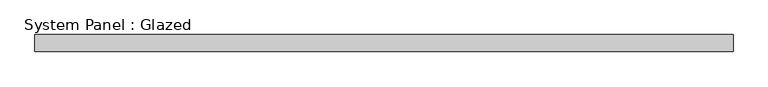
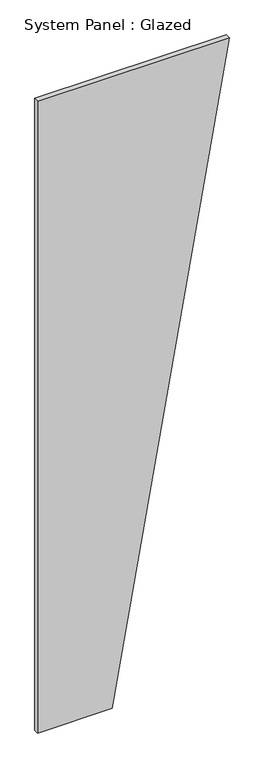
"""IFC4 building model written with IfcOpenShell, lengths in millimetres: plate geometry, System Panel : Glazed."""

from ifc_helpers import new_model, si_unit, frame, origin, place, context, project, spatial, polyline, outline, extrude, source, transform, mapped, element, save


def system_panel_glazed_ce152239(model_context):
    return source(origin(), model_context, "Body", "SweptSolid", [
        extrude(outline(polyline([(0.0, -525.4711374), (0.0, -117.0082603), (3657.6, 525.4711374), (3657.6, -525.4711374), (0.0, -525.4711374)])), frame((0.0, -44.45, 0.0), z_axis=(0.0, 1.0, 0.0), x_axis=(0.0, 0.0, 1.0)), (0.0, 0.0, 1.0), 25.4),
    ])


if __name__ == "__main__":
    model = new_model("IFC4")
    model_context = context("Model", 3, world=origin())
    ifc_project = project(units=[si_unit("LENGTHUNIT", "METRE", prefix="MILLI")], contexts=[model_context])
    site = spatial("IfcSite", under=ifc_project)
    building = spatial("IfcBuilding", under=site)
    placement = place(None, origin())
    system_panel_glazed_shape = system_panel_glazed_ce152239(model_context)
    element("IfcPlate", 1, ObjectType="System Panel : Glazed", at=placement, inside=building, context=model_context, shape_type="MappedRepresentation", body=[
        mapped(system_panel_glazed_shape, transform((0.0, 0.0, 0.0), x_axis=(1.0, 0.0, 0.0), y_axis=(0.0, 1.0, 0.0), z_axis=(0.0, 0.0, 1.0))),
    ])
    save(model, "model.ifc")

# Revit data of these elements
# Type "System Panel : Glazed"
#   Construction Type Id = "GSP4R"
#   Analytic Construction = "1/8 in Pilkington single glazing"
#   Visual Light Transmittance = 0.9
#   Solar Heat Gain Coefficient = 0.86
#   Heat Transfer Coefficient (U) = 1.18115 BTU/(h·ft²·°F)
#   Define Thermal Properties by = 1
# Element 1 (IfcPlate, "System Panel : Glazed")
#   Materials on its faces: "Glass"
# Materials
#   "Glass": class "Glass", colour RGB 0 128 192, transparency 0.75, Description = "Soda Lime Glass", Cost = 0
